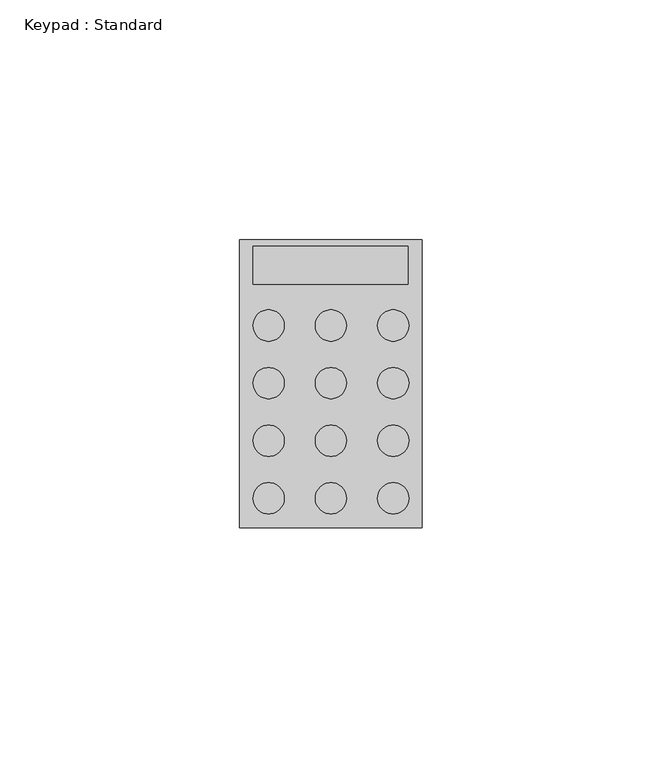
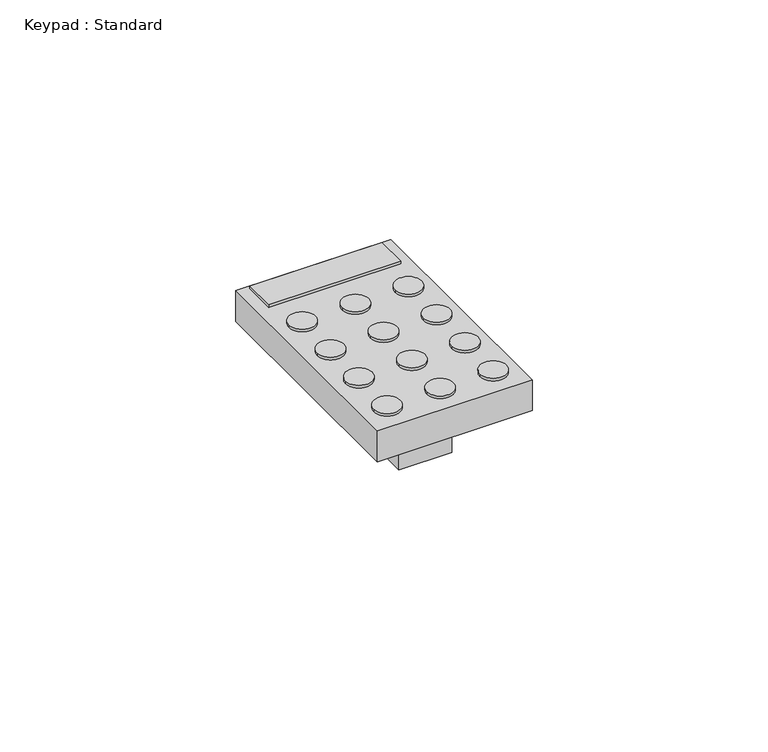
"""IFC4 building model written with IfcOpenShell, lengths in millimetres: proxy geometry, Keypad : Standard."""

from ifc_helpers import new_model, si_unit, point, frame, frame_2d, origin, origin_with_axes, place, context, project, spatial, polyline, circle_curve, trimmed, segment, composite_curve, outline, extrude, source, transform, mapped, element, save


def keypad_standard_b9346bd5(model_context):
    return source(origin(), model_context, "Body", "SweptSolid", [
        extrude(outline(polyline([(19.0, -60.0), (-19.0, -60.0), (-19.0, 0.0), (19.0, 0.0), (19.0, -60.0)])), origin_with_axes(), (0.0, 0.0, 1.0), 8.0),
        extrude(outline(polyline([(6.5, -47.5), (-6.5, -47.5), (-6.5, -12.5), (6.5, -12.5), (6.5, -47.5)])), frame((0.0, 0.0, -14.0), z_axis=(0.0, 0.0, 1.0), x_axis=(1.0, 0.0, 0.0)), (0.0, 0.0, 1.0), 14.0),
        extrude(outline(composite_curve([segment(trimmed(circle_curve(frame_2d((-13.0, -17.8125)), 3.25), [point((-9.75, -17.8125))], [point((-16.25, -17.8125))], False, "CARTESIAN"), True, "CONTINUOUS"), segment(trimmed(circle_curve(frame_2d((-13.0, -17.8125)), 3.25), [point((-16.25, -17.8125))], [point((-9.75, -17.8125))], False, "CARTESIAN"), True, "CONTINUOUS")], self_intersect=False)), frame((0.0, 0.0, 8.0), z_axis=(0.0, 0.0, 1.0), x_axis=(1.0, 0.0, 0.0)), (0.0, 0.0, 1.0), 1.0),
        extrude(outline(composite_curve([segment(trimmed(circle_curve(frame_2d((-13.0, -29.8125)), 3.25), [point((-9.75, -29.8125))], [point((-16.25, -29.8125))], False, "CARTESIAN"), True, "CONTINUOUS"), segment(trimmed(circle_curve(frame_2d((-13.0, -29.8125)), 3.25), [point((-16.25, -29.8125))], [point((-9.75, -29.8125))], False, "CARTESIAN"), True, "CONTINUOUS")], self_intersect=False)), frame((0.0, 0.0, 8.0), z_axis=(0.0, 0.0, 1.0), x_axis=(1.0, 0.0, 0.0)), (0.0, 0.0, 1.0), 1.0),
        extrude(outline(composite_curve([segment(trimmed(circle_curve(frame_2d((-13.0, -41.8125)), 3.25), [point((-9.75, -41.8125))], [point((-16.25, -41.8125))], False, "CARTESIAN"), True, "CONTINUOUS"), segment(trimmed(circle_curve(frame_2d((-13.0, -41.8125)), 3.25), [point((-16.25, -41.8125))], [point((-9.75, -41.8125))], False, "CARTESIAN"), True, "CONTINUOUS")], self_intersect=False)), frame((0.0, 0.0, 8.0), z_axis=(0.0, 0.0, 1.0), x_axis=(1.0, 0.0, 0.0)), (0.0, 0.0, 1.0), 1.0),
        extrude(outline(composite_curve([segment(trimmed(circle_curve(frame_2d((-13.0, -53.8125)), 3.25), [point((-9.75, -53.8125))], [point((-16.25, -53.8125))], False, "CARTESIAN"), True, "CONTINUOUS"), segment(trimmed(circle_curve(frame_2d((-13.0, -53.8125)), 3.25), [point((-16.25, -53.8125))], [point((-9.75, -53.8125))], False, "CARTESIAN"), True, "CONTINUOUS")], self_intersect=False)), frame((0.0, 0.0, 8.0), z_axis=(0.0, 0.0, 1.0), x_axis=(1.0, 0.0, 0.0)), (0.0, 0.0, 1.0), 1.0),
        extrude(outline(composite_curve([segment(trimmed(circle_curve(frame_2d((13.0, -53.8125)), 3.25), [point((16.25, -53.8125))], [point((9.75, -53.8125))], False, "CARTESIAN"), True, "CONTINUOUS"), segment(trimmed(circle_curve(frame_2d((13.0, -53.8125)), 3.25), [point((9.75, -53.8125))], [point((16.25, -53.8125))], False, "CARTESIAN"), True, "CONTINUOUS")], self_intersect=False)), frame((0.0, 0.0, 8.0), z_axis=(0.0, 0.0, 1.0), x_axis=(1.0, 0.0, 0.0)), (0.0, 0.0, 1.0), 1.0),
        extrude(outline(composite_curve([segment(trimmed(circle_curve(frame_2d((0.0, -53.8125)), 3.25), [point((3.25, -53.8125))], [point((-3.25, -53.8125))], False, "CARTESIAN"), True, "CONTINUOUS"), segment(trimmed(circle_curve(frame_2d((0.0, -53.8125)), 3.25), [point((-3.25, -53.8125))], [point((3.25, -53.8125))], False, "CARTESIAN"), True, "CONTINUOUS")], self_intersect=False)), frame((0.0, 0.0, 8.0), z_axis=(0.0, 0.0, 1.0), x_axis=(1.0, 0.0, 0.0)), (0.0, 0.0, 1.0), 1.0),
        extrude(outline(composite_curve([segment(trimmed(circle_curve(frame_2d((0.0, -41.8125)), 3.25), [point((3.25, -41.8125))], [point((-3.25, -41.8125))], False, "CARTESIAN"), True, "CONTINUOUS"), segment(trimmed(circle_curve(frame_2d((0.0, -41.8125)), 3.25), [point((-3.25, -41.8125))], [point((3.25, -41.8125))], False, "CARTESIAN"), True, "CONTINUOUS")], self_intersect=False)), frame((0.0, 0.0, 8.0), z_axis=(0.0, 0.0, 1.0), x_axis=(1.0, 0.0, 0.0)), (0.0, 0.0, 1.0), 1.0),
        extrude(outline(composite_curve([segment(trimmed(circle_curve(frame_2d((0.0, -29.8125)), 3.25), [point((3.25, -29.8125))], [point((-3.25, -29.8125))], False, "CARTESIAN"), True, "CONTINUOUS"), segment(trimmed(circle_curve(frame_2d((0.0, -29.8125)), 3.25), [point((-3.25, -29.8125))], [point((3.25, -29.8125))], False, "CARTESIAN"), True, "CONTINUOUS")], self_intersect=False)), frame((0.0, 0.0, 8.0), z_axis=(0.0, 0.0, 1.0), x_axis=(1.0, 0.0, 0.0)), (0.0, 0.0, 1.0), 1.0),
        extrude(outline(composite_curve([segment(trimmed(circle_curve(frame_2d((0.0, -17.8125)), 3.25), [point((3.25, -17.8125))], [point((-3.25, -17.8125))], False, "CARTESIAN"), True, "CONTINUOUS"), segment(trimmed(circle_curve(frame_2d((0.0, -17.8125)), 3.25), [point((-3.25, -17.8125))], [point((3.25, -17.8125))], False, "CARTESIAN"), True, "CONTINUOUS")], self_intersect=False)), frame((0.0, 0.0, 8.0), z_axis=(0.0, 0.0, 1.0), x_axis=(1.0, 0.0, 0.0)), (0.0, 0.0, 1.0), 1.0),
        extrude(outline(composite_curve([segment(trimmed(circle_curve(frame_2d((13.0, -17.8125)), 3.25), [point((16.25, -17.8125))], [point((9.75, -17.8125))], False, "CARTESIAN"), True, "CONTINUOUS"), segment(trimmed(circle_curve(frame_2d((13.0, -17.8125)), 3.25), [point((9.75, -17.8125))], [point((16.25, -17.8125))], False, "CARTESIAN"), True, "CONTINUOUS")], self_intersect=False)), frame((0.0, 0.0, 8.0), z_axis=(0.0, 0.0, 1.0), x_axis=(1.0, 0.0, 0.0)), (0.0, 0.0, 1.0), 1.0),
        extrude(outline(composite_curve([segment(trimmed(circle_curve(frame_2d((13.0, -29.8125)), 3.25), [point((16.25, -29.8125))], [point((9.75, -29.8125))], False, "CARTESIAN"), True, "CONTINUOUS"), segment(trimmed(circle_curve(frame_2d((13.0, -29.8125)), 3.25), [point((9.75, -29.8125))], [point((16.25, -29.8125))], False, "CARTESIAN"), True, "CONTINUOUS")], self_intersect=False)), frame((0.0, 0.0, 8.0), z_axis=(0.0, 0.0, 1.0), x_axis=(1.0, 0.0, 0.0)), (0.0, 0.0, 1.0), 1.0),
        extrude(outline(composite_curve([segment(trimmed(circle_curve(frame_2d((13.0, -41.8125)), 3.25), [point((16.25, -41.8125))], [point((9.75, -41.8125))], False, "CARTESIAN"), True, "CONTINUOUS"), segment(trimmed(circle_curve(frame_2d((13.0, -41.8125)), 3.25), [point((9.75, -41.8125))], [point((16.25, -41.8125))], False, "CARTESIAN"), True, "CONTINUOUS")], self_intersect=False)), frame((0.0, 0.0, 8.0), z_axis=(0.0, 0.0, 1.0), x_axis=(1.0, 0.0, 0.0)), (0.0, 0.0, 1.0), 1.0),
        extrude(outline(polyline([(16.0429892, -9.21875), (-16.25, -9.21875), (-16.25, -1.2800214), (16.0429892, -1.2800214), (16.0429892, -9.21875)])), frame((0.0, 0.0, 8.0), z_axis=(0.0, 0.0, 1.0), x_axis=(1.0, 0.0, 0.0)), (0.0, 0.0, 1.0), 1.0),
    ])


if __name__ == "__main__":
    model = new_model("IFC4")
    model_context = context("Model", 3, world=origin())
    ifc_project = project(units=[si_unit("LENGTHUNIT", "METRE", prefix="MILLI")], contexts=[model_context])
    site = spatial("IfcSite", under=ifc_project)
    building = spatial("IfcBuilding", under=site)
    placement = place(None, origin())
    keypad_standard_shape = keypad_standard_b9346bd5(model_context)
    element("IfcBuildingElementProxy", 1, Name="Keypad : Standard", ObjectType="Keypad : Standard", at=placement, inside=building, context=model_context, shape_type="MappedRepresentation", body=[
        mapped(keypad_standard_shape, transform((0.0, 0.0, 0.0), x_axis=(1.0, 0.0, 0.0), y_axis=(0.0, 1.0, 0.0), z_axis=(0.0, 0.0, 1.0))),
    ])
    save(model, "model.ifc")

# Revit data of these elements
# Type "Keypad : Standard"
#   Type Mark = "Keypad"
#   Classification.OmniClass.23.Number = "23-29 11 27 13"
#   Classification.OmniClass.23.Description = "Security Keypad"
#   COBie.Type.CreatedBy = "info@mma.ie"
#   COBie.Type.CreatedOn = "2017-07-26T09:25:07"
#   COBie.Type.Name = "Keypad"
#   COBie.Type.Category = "23-29 11 27 13 : Security Keypad"
#   COBie.Type.Description = "Keypad_Standard"
#   COBie.Type.AssetType = "Fixed"
#   COBie.Type.Manufacturer = ""
#   COBie.Type.ModelNumber = ""
#   Keynote = "28 13 00.D"
#   COBie.Type.ReplacementCost = 0
#   K.Width = 38 mm
#   K.Height = 60 mm
#   K.Depth = 22 mm
#   Default Elevation = 1200 mm
#   COBie.Type = yes
#   URL = ""
#   Model = ""
#   Manufacturer = ""
